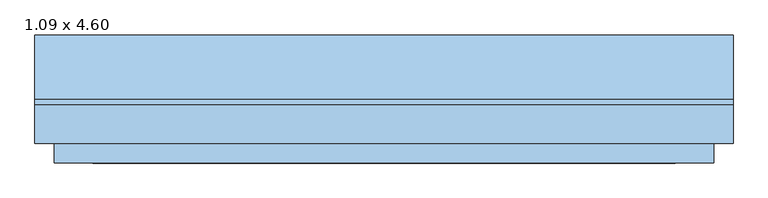
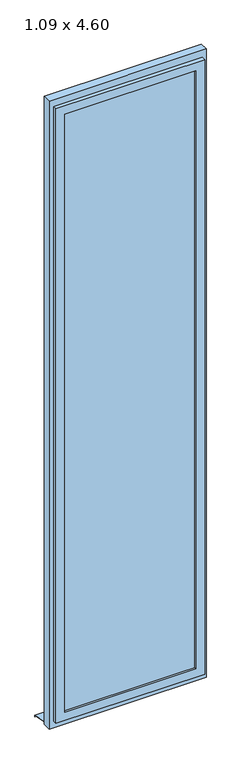
"""IFC4 building model written with IfcOpenShell, lengths in millimetres: window geometry, Fenstertür 1-flg : 1.09 x 4.60."""

from ifc_helpers import new_model, si_unit, frame, origin, place, context, project, spatial, polyline, outline, extrude, faceted_brep, source, transform, mapped, element, save


def window_1_09_x_4_60_b0627fdd(model_context):
    return source(origin(), model_context, "Body", "SolidModel", [
        extrude(outline(polyline([(4600.0, 545.0), (4600.0, -545.0), (0.0, -545.0), (0.0, 545.0), (4600.0, 545.0)]), holes=[polyline([(4520.0, 485.0), (80.0, 485.0), (80.0, -485.0), (4520.0, -485.0), (4520.0, 485.0)])]), frame((0.0, -80.0, 0.0), z_axis=(0.0, 1.0, 0.0), x_axis=(0.0, 0.0, 1.0)), (0.0, 0.0, 1.0), 60.0),
        faceted_brep([(515.0, -80.0, 4550.0), (515.0, -110.0, 4550.0), (515.0, -110.0, 50.0), (515.0, -80.0, 50.0), (-515.0, -110.0, 4550.0), (-515.0, -110.0, 50.0), (455.0, -110.0, 110.0), (-455.0, -110.0, 110.0), (-455.0, -110.0, 4490.0), (455.0, -110.0, 4490.0), (-515.0, -80.0, 50.0), (-515.0, -80.0, 4550.0), (485.0, -80.0, 4520.0), (-485.0, -80.0, 4520.0), (-485.0, -80.0, 80.0), (485.0, -80.0, 80.0), (485.0, -50.0, 4520.0), (485.0, -50.0, 80.0), (-485.0, -50.0, 80.0), (-485.0, -50.0, 4520.0), (455.0, -50.0, 4490.0), (-455.0, -50.0, 4490.0), (-455.0, -50.0, 110.0), (455.0, -50.0, 110.0)], [[[0, 1, 2, 3]], [[1, 4, 5, 2], [6, 7, 8, 9]], [[3, 2, 5, 10]], [[3, 10, 11, 0], [12, 13, 14, 15]], [[16, 12, 15, 17]], [[17, 15, 14, 18]], [[17, 18, 19, 16], [20, 21, 22, 23]], [[9, 20, 23, 6]], [[6, 23, 22, 7]], [[10, 5, 4, 11]], [[18, 14, 13, 19]], [[7, 22, 21, 8]], [[11, 4, 1, 0]], [[19, 13, 12, 16]], [[8, 21, 20, 9]]]),
        extrude(outline(polyline([(-9.9778457, 20.0), (90.0, 0.0), (90.0, -10.0), (88.0, -10.0), (88.0, -1.6395366), (-10.1759277, 18.0), (-20.0, 18.0), (-20.0, 20.0), (-9.9778457, 20.0)])), frame((-545.0, 0.0, 0.0), z_axis=(1.0, 0.0, 0.0), x_axis=(0.0, 1.0, 0.0)), (0.0, 0.0, 1.0), 1090.0),
        extrude(outline(polyline([(455.0, -95.0), (-455.0, -95.0), (-455.0, -65.0), (455.0, -65.0), (455.0, -95.0)])), frame((0.0, 0.0, 110.0), z_axis=(0.0, 0.0, 1.0), x_axis=(1.0, 0.0, 0.0)), (0.0, 0.0, 1.0), 4380.0),
    ])


if __name__ == "__main__":
    model = new_model("IFC4")
    model_context = context("Model", 3, world=origin())
    ifc_project = project(units=[si_unit("LENGTHUNIT", "METRE", prefix="MILLI")], contexts=[model_context])
    site = spatial("IfcSite", under=ifc_project)
    building = spatial("IfcBuilding", under=site)
    placement = place(None, origin())
    window_1_09_x_4_60_shape = window_1_09_x_4_60_b0627fdd(model_context)
    element("IfcWindow", 1, ObjectType="Fenstertür 1-flg : 1.09 x 4.60", at=placement, inside=building, context=model_context, shape_type="MappedRepresentation", body=[
        mapped(window_1_09_x_4_60_shape, transform((0.0, 0.0, 0.0), x_axis=(1.0, 0.0, 0.0), y_axis=(0.0, 1.0, 0.0), z_axis=(0.0, 0.0, 1.0))),
    ])
    save(model, "model.ifc")

# Revit data of these elements
# Type "Fenstertür 1-flg : 1.09 x 4.60"
#   Type Mark = "53"
#   Operation = "SinglePanel"
#   Construction Type Id = "SGL"
#   Keynote = "16.05.01"
#   Analytic Construction = "Große Fenster mit Einfachverglasung"
#   Visual Light Transmittance = 0.9
#   Solar Heat Gain Coefficient = 0.86
#   Rough Width = 1.090 m
#   Rough Height = 4.600 m
#   Heat Transfer Coefficient (U) = 5.5617 W/(m²·K)
#   Rahmentiefe = 0.060 m
#   Rahmenhöhe unten = 0.080 m
#   Höhe oberer  Rahmen = 0.080 m
#   Rahmenbreite = 0.060 m
#   Height = 4.600 m
#   Tiefe Flügel = 0.060 m
#   Flügelbreite = 0.060 m
#   Einbautiefe (von außen) [instance default] = 0.080 m
#   Width = 1.090 m
#   Sichtbarkeit Sturzlinien [instance default] = yes
#   Öffnungsrichtung oben [instance default] = yes
#   Öffnungsrichtung in Draufsicht anzeigen [instance default] = yes
#   Drehflügel 1 [instance default] = yes
#   Bild [instance default] = none
#   Glas [instance default] = none
#   Fensterflügel [instance default] = none
#   Äußere Fensterbank [instance default] = none
#   Wall Closure = (empty or 0)
# Element 1 (IfcWindow, "Fenstertür 1-flg : 1.09 x 4.60")
#   Materials on its faces: "Kunststoff - Weiß", "Glas"
# Materials
#   "Kunststoff - Weiß": class "Kunststoff", colour RGB 249 249 249, transparency 0, Cost = 0
#   "Glas": class "Glas", colour RGB 0 0 255, transparency 0.75, Comments = "Render-Darstellung nicht aktualisiert ", Cost = 0
